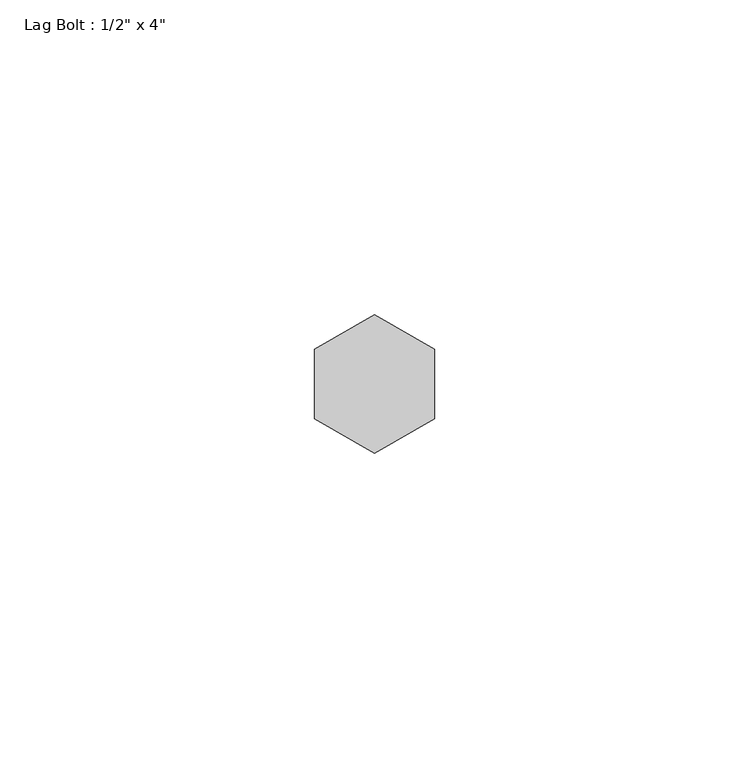
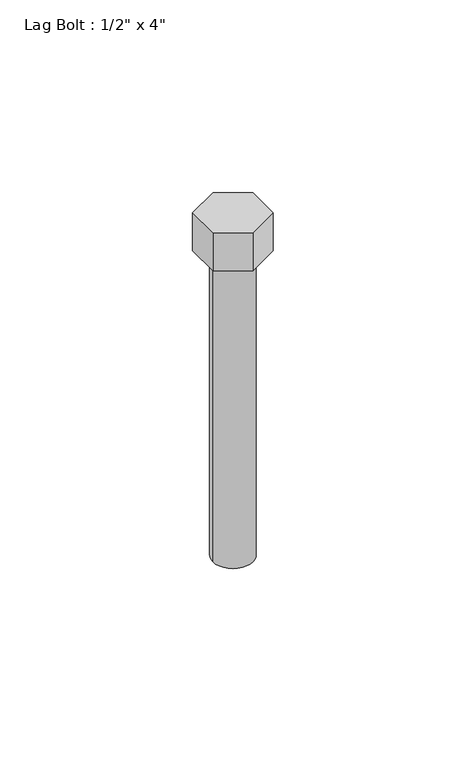
"""IFC4 building model written with IfcOpenShell, lengths in millimetres: proxy geometry."""

from ifc_helpers import new_model, si_unit, point, frame, origin, origin_with_axes, origin_2d, place, context, project, spatial, polyline, circle_curve, trimmed, segment, composite_curve, outline, extrude, source, transform, mapped, element, save


def proxy_7df0dc6f(model_context):
    return source(origin(), model_context, "Body", "SweptSolid", [
        extrude(outline(polyline([(-9.525, 5.4992613), (0.0, 10.9985226), (9.525, 5.4992613), (9.525, -5.4992613), (0.0, -10.9985226), (-9.525, -5.4992613), (-9.525, 5.4992613)])), origin_with_axes(), (0.0, 0.0, 1.0), 12.7),
        extrude(outline(composite_curve([segment(trimmed(circle_curve(origin_2d(), 6.35), [point((-6.35, 0.0))], [point((6.35, 0.0))], False, "CARTESIAN"), True, "CONTINUOUS"), segment(trimmed(circle_curve(origin_2d(), 6.35), [point((6.35, 0.0))], [point((-6.35, 0.0))], False, "CARTESIAN"), True, "CONTINUOUS")], self_intersect=False)), frame((0.0, 0.0, -101.6), z_axis=(0.0, 0.0, 1.0), x_axis=(1.0, 0.0, 0.0)), (0.0, 0.0, 1.0), 101.6),
    ])


if __name__ == "__main__":
    model = new_model("IFC4")
    model_context = context("Model", 3, world=origin())
    ifc_project = project(units=[si_unit("LENGTHUNIT", "METRE", prefix="MILLI")], contexts=[model_context])
    site = spatial("IfcSite", under=ifc_project)
    building = spatial("IfcBuilding", under=site)
    placement = place(None, origin())
    proxy_shape = proxy_7df0dc6f(model_context)
    element("IfcBuildingElementProxy", 1, Name="Lag Bolt : 1/2\" x 4\"", ObjectType="Lag Bolt : 1/2\" x 4\"", at=placement, inside=building, context=model_context, shape_type="MappedRepresentation", body=[
        mapped(proxy_shape, transform((0.0, 0.0, 0.0), x_axis=(1.0, 0.0, 0.0), y_axis=(0.0, 1.0, 0.0), z_axis=(0.0, 0.0, 1.0))),
    ])
    save(model, "model.ifc")

# Revit data of these elements
# Type "Lag Bolt : 1/2\" x 4\""
#   Thickness_of_Substrate [instance default] = 0' - 1"
#   Side = 0' - 0 111/256"
#   Radius = 0' - 0 1/4"
#   Length = 0' - 4"
#   Head Size = 0' - 0 3/4"
#   Head Radius = 0' - 0 3/8"
#   Head Height = 0' - 0 1/2"
#   Diameter = 0' - 0 1/2"
#   Default Elevation = 4' - 0"
#   Nut_Visibility [instance default] = yes
#   Bolt Material (Size) [instance default] = 1" GALV. LAG BOLT (LENGTH = 1/2" SHY OF GLULAM DEPTH) -  (GALV. THRU BOLT IF PLATE ON OPP. SIDE OF STRUCT MEMBER)
# Element 1 (IfcBuildingElementProxy, "Lag Bolt : 1/2\" x 4\"")
#   Nut_Visibility = no
#   Bolt Material (Size) = 1/2 LAG BOLTS 24" O.C.
#   Materials on its faces: "1/2 LAG BOLTS 24\" O.C."
# Materials
#   "1\" GALV. LAG BOLT (LENGTH = 1/2\" SHY OF GLULAM DEPTH) -  (GALV. THRU BOLT IF PLATE ON OPP. SIDE OF STRUCT MEMBER)": class "Generic", colour RGB 120 120 120, transparency 0, Cost = 0
#   "1/2 LAG BOLTS 24\" O.C.": class "Generic", colour RGB 120 120 120, transparency 0, Cost = 0
